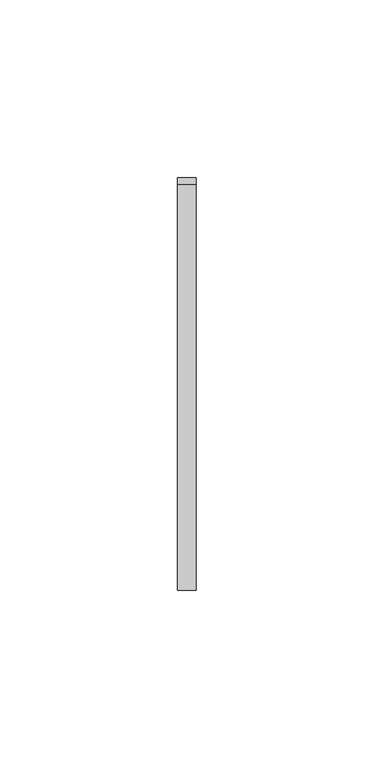
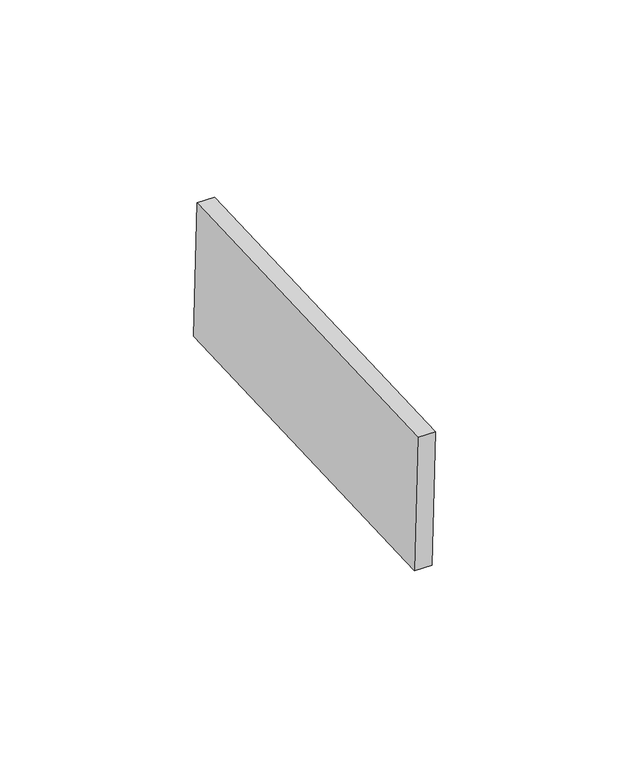
"""IFC4 building model written with IfcOpenShell, lengths in millimetres: proxy geometry, Inner panel:Inner panel:1:Inner panel:1 : Inner panel:Inner panel:300324:2:Inner panel:1:Inner panel:1 : Inner panel:Inner panel:300324:2 : Inner panel:Inner panel:1:Inner panel:1 : Inner panel:Inner panel:300324:300043:52 : Inner panel:Inner panel:1:Inner panel:1 : Inner panel:Inner panel:300324:2:Inner panel:1:Inner panel:1 : Inner panel:Inner panel:300324:2 : Inner panel:Inner panel:1:Inner panel:1 : Inner panel:Inner panel:300324:300043:308120."""

from ifc_helpers import new_model, si_unit, frame, origin, place, context, project, spatial, polyline, outline, extrude, source, transform, mapped, element, save


def generic_models_6e5a32b0(model_context):
    return source(origin(), model_context, "Body", "SweptSolid", [
        extrude(outline(polyline([(0.0, -114.2999999), (0.0, 0.0), (5.2138089, 0.0), (5.2138089, -114.2999999), (0.0, -114.2999999)])), frame((593123.795117, -566950.1308393, 8857.6957503), z_axis=(0.0, -0.04163054471215927, 0.9991330730923529), x_axis=(-1.0, 0.0, 0.0)), (0.0, 0.0, 1.0), 43.2233908),
    ])


if __name__ == "__main__":
    model = new_model("IFC4")
    model_context = context("Model", 3, world=origin())
    ifc_project = project(units=[si_unit("LENGTHUNIT", "METRE", prefix="MILLI")], contexts=[model_context])
    site = spatial("IfcSite", under=ifc_project)
    building = spatial("IfcBuilding", under=site)
    placement = place(None, origin())
    generic_models_shape = generic_models_6e5a32b0(model_context)
    element("IfcBuildingElementProxy", 1, Name="Inner panel:Inner panel:1:Inner panel:1 : Inner panel:Inner panel:300324:2:Inner panel:1:Inner panel:1 : Inner panel:Inner panel:300324:2 : Inner panel:Inner panel:1:Inner panel:1 : Inner panel:Inner panel:300324:300043:52 : Inner panel:Inner panel:1:Inner panel:1 : Inner panel:Inner panel:300324:2:Inner panel:1:Inner panel:1 : Inner panel:Inner panel:300324:2 : Inner panel:Inner panel:1:Inner panel:1 : Inner panel:Inner panel:300324:300043:308120", ObjectType="Inner panel:Inner panel:1:Inner panel:1 : Inner panel:Inner panel:300324:2:Inner panel:1:Inner panel:1 : Inner panel:Inner panel:300324:2 : Inner panel:Inner panel:1:Inner panel:1 : Inner panel:Inner panel:300324:300043:52 : Inner panel:Inner panel:1:Inner panel:1 : Inner panel:Inner panel:300324:2:Inner panel:1:Inner panel:1 : Inner panel:Inner panel:300324:2 : Inner panel:Inner panel:1:Inner panel:1 : Inner panel:Inner panel:300324:300043:308120", at=placement, inside=building, context=model_context, shape_type="MappedRepresentation", body=[
        mapped(generic_models_shape, transform((0.0, 0.0, 0.0), x_axis=(1.0, 0.0, 0.0), y_axis=(0.0, 1.0, 0.0), z_axis=(0.0, 0.0, 1.0))),
    ])
    save(model, "model.ifc")

# Revit data of these elements
# Type "Inner panel:Inner panel:1:Inner panel:1 : Inner panel:Inner panel:300324:2:Inner panel:1:Inner panel:1 : Inner panel:Inner panel:300324:2 : Inner panel:Inner panel:1:Inner panel:1 : Inner panel:Inner panel:300324:300043:52 : Inner panel:Inner panel:1:Inner panel:1 : Inner panel:Inner panel:300324:2:Inner panel:1:Inner panel:1 : Inner panel:Inner panel:300324:2 : Inner panel:Inner panel:1:Inner panel:1 : Inner panel:Inner panel:300324:300043:308120"
#   NameOverride = "Inner panel:Inner panel:1:Inner panel:1 : Inner panel:Inner panel:300324:2:Inner panel:1:Inner panel:1 : Inner panel:Inner panel:300324:2 : Inner panel:Inner panel:1:Inner panel:1 : Inner panel:Inner panel:300324:300043:308120"
#   ObjectTypeOverride = "Inner panel:1:Inner panel:1 : Inner panel:Inner panel:300324:2 : Inner panel:Inner panel:1:Inner panel:1 : Inner panel:Inner panel:300324:300043"
#   Reference = "Inner panel"
#   Tag = "308120"
# Element 1 (IfcBuildingElementProxy, "Inner panel:Inner panel:1:Inner panel:1 : Inner panel:Inner panel:300324:2:Inner panel:1:Inner panel:1 : Inner panel:Inner panel:300324:2 : Inner panel:Inner panel:1:Inner panel:1 : Inner panel:Inner panel:300324:300043:52 : Inner panel:Inner panel:1:Inner panel:1 : Inner panel:Inner panel:300324:2:Inner panel:1:Inner panel:1 : Inner panel:Inner panel:300324:2 : Inner panel:Inner panel:1:Inner panel:1 : Inner panel:Inner panel:300324:300043:308120")
#   Materials on its faces: "SLIDING CLIP"
# Materials
#   "SLIDING CLIP": class "Generic", colour RGB 120 120 120, transparency 0, Cost = 0
